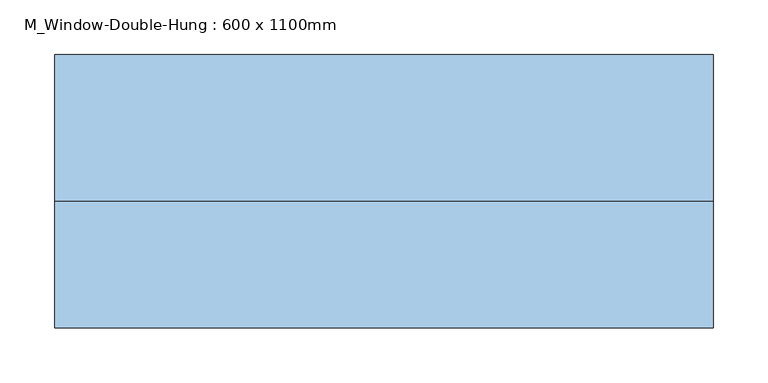
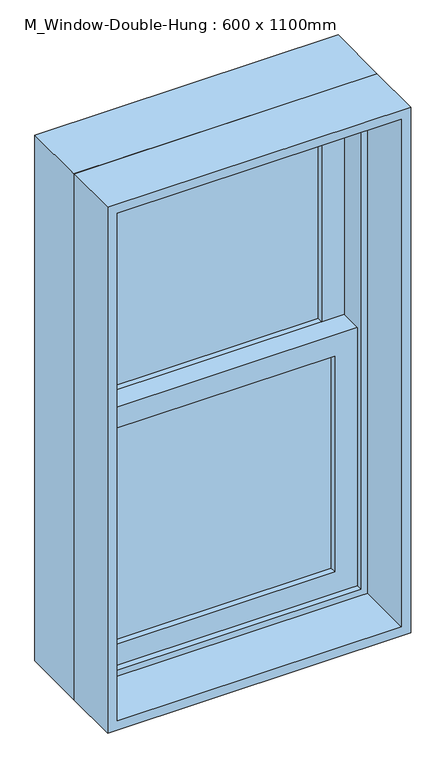
"""IFC4 building model written with IfcOpenShell, lengths in millimetres: window geometry, M_Window-Double-Hung : 600 x 1100mm."""

import ifcopenshell
import ifcopenshell.guid

model = None  # the IFC model being written
_history = None  # IfcOwnerHistory: only IFC2X3 demands one
_inside = {}  # id of a spatial element -> (the spatial element, [elements in it])
_under = {}  # id of a project, library or spatial element -> (it, [spatial elements below it])
_declared = {}  # id of a project -> (the project, [libraries it declares])
_typed = {}  # id of a type object -> (the type object, [elements of that type])
_made_of = {}  # id of a material, layer set ... -> (it, [elements and type objects made of it])


def new_model(schema):
    """Start an empty IFC model of exactly this schema.

    Asked for "IFC4X3", IfcOpenShell would pick the latest addendum, in which some entities
    have other attributes; the version numbers below select the first issue.
    IFC2X3 requires an IfcOwnerHistory on every rooted entity: one is made here for all.
    """
    global model, _history
    if schema == "IFC4X3":
        model = ifcopenshell.file(schema_version=(4, 3, 0, 0))
    else:
        model = ifcopenshell.file(schema=schema)
    _inside.clear()
    _under.clear()
    _declared.clear()
    _typed.clear()
    _made_of.clear()
    _history = None
    if model.schema == "IFC2X3":
        org = make("IfcOrganization", Name="unknown")
        user = make(
            "IfcPersonAndOrganization",
            ThePerson=make("IfcPerson", FamilyName="unknown"),
            TheOrganization=org,
        )
        app = make(
            "IfcApplication",
            ApplicationDeveloper=org,
            Version="unknown",
            ApplicationFullName="unknown",
            ApplicationIdentifier="unknown",
        )
        _history = make(
            "IfcOwnerHistory",
            OwningUser=user,
            OwningApplication=app,
            ChangeAction="ADDED",
            CreationDate=0,
        )
    return model


def make(cls, **values):
    """One entity of the class cls with the attributes given. An attribute that is None is left unset."""
    return model.create_entity(
        cls, **{name: value for name, value in values.items() if value is not None}
    )


def rooted(cls, **values):
    """An entity with a GlobalId (a new one), such as an element, a storey or a relation."""
    return make(cls, GlobalId=ifcopenshell.guid.new(), OwnerHistory=_history, **values)


def si_unit(unit_type, name, prefix=None):
    """IfcSIUnit, for example si_unit("LENGTHUNIT", "METRE", prefix="MILLI")."""
    return make("IfcSIUnit", UnitType=unit_type, Prefix=prefix, Name=name)


def assignment(units):
    """IfcUnitAssignment: the units of a project."""
    return None if units is None else make("IfcUnitAssignment", Units=units)


def point(xyz):
    """IfcCartesianPoint."""
    return None if xyz is None else make("IfcCartesianPoint", Coordinates=xyz)


def direction(xyz):
    """IfcDirection."""
    return None if xyz is None else make("IfcDirection", DirectionRatios=xyz)


def frame(location, z_axis=None, x_axis=None):
    """IfcAxis2Placement3D, a coordinate frame: its origin and axes. An axis left out is left unset."""
    return make(
        "IfcAxis2Placement3D",
        Location=point(location),
        Axis=direction(z_axis),
        RefDirection=direction(x_axis),
    )


def origin():
    """The frame at (0, 0, 0) with its axes left unset."""
    return frame((0.0, 0.0, 0.0))


def place(relative_to, where):
    """IfcLocalPlacement: puts the frame where relative to a parent placement (None: the world)."""
    return make(
        "IfcLocalPlacement", PlacementRelTo=relative_to, RelativePlacement=where
    )


def context(
    kind, dimensions, precision=None, world=None, true_north=None, identifier=None
):
    """IfcGeometricRepresentationContext, for example the 3D "Model" context."""
    return make(
        "IfcGeometricRepresentationContext",
        ContextIdentifier=identifier,
        ContextType=kind,
        CoordinateSpaceDimension=dimensions,
        Precision=precision,
        WorldCoordinateSystem=world,
        TrueNorth=true_north,
    )


def project(units=None, contexts=None):
    """IfcProject with its units and contexts."""
    return rooted(
        "IfcProject",
        Name="project",
        RepresentationContexts=contexts,
        UnitsInContext=assignment(units),
    )


def spatial(cls, under=None, at=None, **own):
    """A site, building, storey or space (cls), placed at a placement, below another one or the project."""
    s = rooted(cls, ObjectPlacement=at, **own)
    if under is not None:
        _under.setdefault(under.id(), (under, []))[1].append(s)
    return s


def polyline(points):
    """IfcPolyline through the points."""
    return make("IfcPolyline", Points=[point(p) for p in points])


def outline(outer, holes=None, kind="AREA"):
    """IfcArbitraryClosedProfileDef: a profile drawn as a closed curve; with holes, ...WithVoids."""
    if holes is None:
        return make("IfcArbitraryClosedProfileDef", ProfileType=kind, OuterCurve=outer)
    return make(
        "IfcArbitraryProfileDefWithVoids",
        ProfileType=kind,
        OuterCurve=outer,
        InnerCurves=holes,
    )


def extrude(swept, where, along, depth):
    """IfcExtrudedAreaSolid: the profile swept, set in the frame where, extruded along a direction by depth."""
    return make(
        "IfcExtrudedAreaSolid",
        SweptArea=swept,
        Position=where,
        ExtrudedDirection=direction(along),
        Depth=depth,
    )


def shape(context_of_items, identifier, shape_type, items):
    """IfcShapeRepresentation: the items that make up one representation, for example the "Body"."""
    return make(
        "IfcShapeRepresentation",
        ContextOfItems=context_of_items,
        RepresentationIdentifier=identifier,
        RepresentationType=shape_type,
        Items=items,
    )


def source(mapping_origin, context_of_items, identifier, shape_type, items):
    """IfcRepresentationMap: a shape defined once, which mapped items show again and again."""
    return make(
        "IfcRepresentationMap",
        MappingOrigin=mapping_origin,
        MappedRepresentation=shape(context_of_items, identifier, shape_type, items),
    )


def transform(
    local_origin,
    x_axis=None,
    y_axis=None,
    z_axis=None,
    scale=None,
    scale2=None,
    scale3=None,
    uniform=True,
):
    """IfcCartesianTransformationOperator3D, or its non-uniform kind. x_axis, y_axis, z_axis: its Axis1, 2, 3."""
    if uniform:
        return make(
            "IfcCartesianTransformationOperator3D",
            Axis1=direction(x_axis),
            Axis2=direction(y_axis),
            LocalOrigin=point(local_origin),
            Scale=scale,
            Axis3=direction(z_axis),
        )
    return make(
        "IfcCartesianTransformationOperator3DnonUniform",
        Axis1=direction(x_axis),
        Axis2=direction(y_axis),
        LocalOrigin=point(local_origin),
        Scale=scale,
        Axis3=direction(z_axis),
        Scale2=scale2,
        Scale3=scale3,
    )


def mapped(mapping_source, mapping_target):
    """IfcMappedItem: shows the shape of a source again, moved by a transform."""
    return make(
        "IfcMappedItem", MappingSource=mapping_source, MappingTarget=mapping_target
    )


def made_of(thing, what):
    """Note that an element or type object is made of a material, layer set ...; save() writes the relation."""
    if what is not None:
        _made_of.setdefault(what.id(), (what, []))[1].append(thing)
    return thing


def element(
    cls,
    number,
    at=None,
    inside=None,
    cuts=None,
    type_object=None,
    material=None,
    context=None,
    identifier="Body",
    shape_type=None,
    held_by="IfcProductDefinitionShape",
    body=None,
    shapes=None,
    **own,
):
    """One element of the class cls, such as IfcWall. Its Tag is "e" and its number.

    at: its placement. inside: the storey or other place that contains it. cuts: it is an
    opening in that element (IfcRelVoidsElement). A single representation is given by context,
    identifier, shape_type and body (its items); several are given by shapes. held_by: the class
    of the entity that holds the representations. save() writes the other relations.
    """
    e = rooted(cls, Tag="e%d" % number, ObjectPlacement=at, **own)
    if body is not None:
        shapes = [shape(context, identifier, shape_type, body)]
    if shapes is not None:
        e.Representation = make(held_by, Representations=shapes)
    if inside is not None:
        _inside.setdefault(inside.id(), (inside, []))[1].append(e)
    if cuts is not None:
        rooted(
            "IfcRelVoidsElement", RelatingBuildingElement=cuts, RelatedOpeningElement=e
        )
    if type_object is not None:
        _typed.setdefault(type_object.id(), (type_object, []))[1].append(e)
    return made_of(e, material)


def aggregate(whole, parts):
    """IfcRelAggregates: a whole, such as a stair, and the parts it consists of."""
    return rooted("IfcRelAggregates", RelatingObject=whole, RelatedObjects=parts)


def save(model, path):
    """Write the relations noted so far, then the file.

    IfcRelAggregates (storeys below a building ...), IfcRelContainedInSpatialStructure (elements
    in a storey), IfcRelDefinesByType, IfcRelAssociatesMaterial and IfcRelDeclares: one each for
    every whole, place, type object, material and project.
    """
    for whole, parts in _under.values():
        aggregate(whole, parts)
    for where, things in _inside.values():
        rooted(
            "IfcRelContainedInSpatialStructure",
            RelatedElements=things,
            RelatingStructure=where,
        )
    for kind, things in _typed.values():
        rooted("IfcRelDefinesByType", RelatedObjects=things, RelatingType=kind)
    for what, things in _made_of.values():
        rooted("IfcRelAssociatesMaterial", RelatedObjects=things, RelatingMaterial=what)
    for by, libraries in _declared.values():
        rooted("IfcRelDeclares", RelatingContext=by, RelatedDefinitions=libraries)
    model.write(path)


def m_window_double_hung_600_x_1100mm_c7e90a65(model_context):
    return source(origin(), model_context, "Body", "SweptSolid", [
        extrude(outline(polyline([(223.8, 45.15), (223.8, 38.8), (-223.8, 38.8), (-223.8, 45.15), (223.8, 45.15)])), frame((0.0, 0.0, 990.6), z_axis=(0.0, 0.0, 1.0), x_axis=(1.0, 0.0, 0.0)), (0.0, 0.0, 1.0), 451.575),
        extrude(outline(polyline([(-223.8, 32.45), (223.8, 32.45), (223.8, 26.1), (-223.8, 26.1), (-223.8, 32.45)])), frame((0.0, 0.0, 990.6), z_axis=(0.0, 0.0, 1.0), x_axis=(1.0, 0.0, 0.0)), (0.0, 0.0, 1.0), 451.575),
        extrude(outline(polyline([(223.8, 89.6), (223.8, 83.25), (-223.8, 83.25), (-223.8, 89.6), (223.8, 89.6)])), frame((0.0, 0.0, 1486.625), z_axis=(0.0, 0.0, 1.0), x_axis=(1.0, 0.0, 0.0)), (0.0, 0.0, 1.0), 451.575),
        extrude(outline(polyline([(-223.8, 76.9), (223.8, 76.9), (223.8, 70.55), (-223.8, 70.55), (-223.8, 76.9)])), frame((0.0, 0.0, 1486.625), z_axis=(0.0, 0.0, 1.0), x_axis=(1.0, 0.0, 0.0)), (0.0, 0.0, 1.0), 451.575),
        extrude(outline(polyline([(1486.625, -268.25), (946.15, -268.25), (946.15, 268.25), (1486.625, 268.25), (1486.625, -268.25)]), holes=[polyline([(1442.175, 223.8), (990.6, 223.8), (990.6, -223.8), (1442.175, -223.8), (1442.175, 223.8)])]), frame((0.0, 13.4, 0.0), z_axis=(0.0, 1.0, 0.0), x_axis=(0.0, 0.0, 1.0)), (0.0, 0.0, 1.0), 44.45),
        extrude(outline(polyline([(1982.65, -268.25), (1442.175, -268.25), (1442.175, 268.25), (1982.65, 268.25), (1982.65, -268.25)]), holes=[polyline([(1938.2, 223.8), (1486.625, 223.8), (1486.625, -223.8), (1938.2, -223.8), (1938.2, 223.8)])]), frame((0.0, 57.85, 0.0), z_axis=(0.0, 1.0, 0.0), x_axis=(0.0, 0.0, 1.0)), (0.0, 0.0, 1.0), 44.45),
        extrude(outline(polyline([(2014.4, -300.0), (914.4, -300.0), (914.4, 300.0), (2014.4, 300.0), (2014.4, -300.0)]), holes=[polyline([(1982.65, 268.25), (946.15, 268.25), (946.15, -268.25), (1982.65, -268.25), (1982.65, 268.25)])]), frame((0.0, 0.7, 0.0), z_axis=(0.0, 1.0, 0.0), x_axis=(0.0, 0.0, 1.0)), (0.0, 0.0, 1.0), 133.35),
        extrude(outline(polyline([(2014.4, 300.0), (2014.4, -300.0), (914.4, -300.0), (914.4, 300.0), (2014.4, 300.0)]), holes=[polyline([(1995.35, 280.95), (933.45, 280.95), (933.45, -280.95), (1995.35, -280.95), (1995.35, 280.95)])]), frame((0.0, -115.0, 0.0), z_axis=(0.0, 1.0, 0.0), x_axis=(0.0, 0.0, 1.0)), (0.0, 0.0, 1.0), 115.7),
    ])


if __name__ == "__main__":
    model = new_model("IFC4")
    model_context = context("Model", 3, world=origin())
    ifc_project = project(units=[si_unit("LENGTHUNIT", "METRE", prefix="MILLI")], contexts=[model_context])
    site = spatial("IfcSite", under=ifc_project)
    building = spatial("IfcBuilding", under=site)
    placement = place(None, origin())
    m_window_double_hung_600_x_1100mm_shape = m_window_double_hung_600_x_1100mm_c7e90a65(model_context)
    element("IfcWindow", 1, ObjectType="M_Window-Double-Hung : 600 x 1100mm", at=placement, inside=building, context=model_context, shape_type="MappedRepresentation", body=[
        mapped(m_window_double_hung_600_x_1100mm_shape, transform((0.0, 0.0, 0.0), x_axis=(1.0, 0.0, 0.0), y_axis=(0.0, 1.0, 0.0), z_axis=(0.0, 0.0, 1.0))),
    ])
    save(model, "model.ifc")

# Revit data of these elements
# Type "M_Window-Double-Hung : 600 x 1100mm"
#   Type Mark = "19"
#   Fire Rating = "0.5h"
#   Construction Type Id = "DG-DR"
#   Assembly Code = "B2020100"
#   Analytic Construction = "Double glazing - domestic"
#   Wall Thickness [instance default] = 15 cm
#   Window Inset [instance default] = 0 cm
#   Visual Light Transmittance = 0.81
#   Thermal Resistance (R) = 0.319569 (m²·K)/W
#   Solar Heat Gain Coefficient = 0.76
#   Muntin Width = 44.76 cm
#   Muntin Height = 45.1575 cm
#   Interior Wall Closure [instance default] = 3.57 cm
#   Rough Width = 61.5 cm
#   Rough Height = 111.5 cm
#   Frame Extension [instance default] = 3.175 cm
#   Exterior Wall Closure [instance default] = 1.27 cm
#   Extension Jamb [instance default] = 3.57 cm
#   Heat Transfer Coefficient (U) = 3.12929 W/(m²·K)
#   Height = 110 cm
#   Width = 60 cm
#   Top Muntin Visibility = yes
#   Indicator Visibility [instance default] = yes
#   Extension Jamb Visibility [instance default] = yes
#   Interior Trim Visibility [instance default] = yes
#   Exterior Trim Visibility [instance default] = yes
#   Bottom Muntin Visibility = yes
#   Muntin Pattern = M_Muntin Pattern_2x2 : M_Muntin Pattern_2x2
#   Interior Trim Material = Wood - Stained
#   Interior Trim = M_Trim-Window-Interior-Flat : Picture Frame
#   Exterior Trim Material = Clad - White
#   Exterior Trim = M_Trim-Window-Exterior-Flat : with Sill
#   Glass Panel Material = Glass
#   Exterior Frame Material = Clad - White
#   Interior Frame Material = Wood - Stained
#   Wall Closure = (empty or 0)
# Element 1 (IfcWindow, "M_Window-Double-Hung : 600 x 1100mm")
#   Wall Thickness = 23 cm
#   Extension Jamb = 11.57 cm
#   Materials on its faces: "Wood - Stained", "Glass", "Clad - White"
# Materials
#   "Wood - Stained": class "Wood", colour RGB 224 178 126, transparency 0, Cost = 0
#   "Clad - White": class "Wood", colour RGB 242 242 238, transparency 0, Cost = 0
#   "Glass": class "Glass", colour RGB 0 128 192, transparency 0.9, Description = "Soda Lime Glass", Cost = 0
